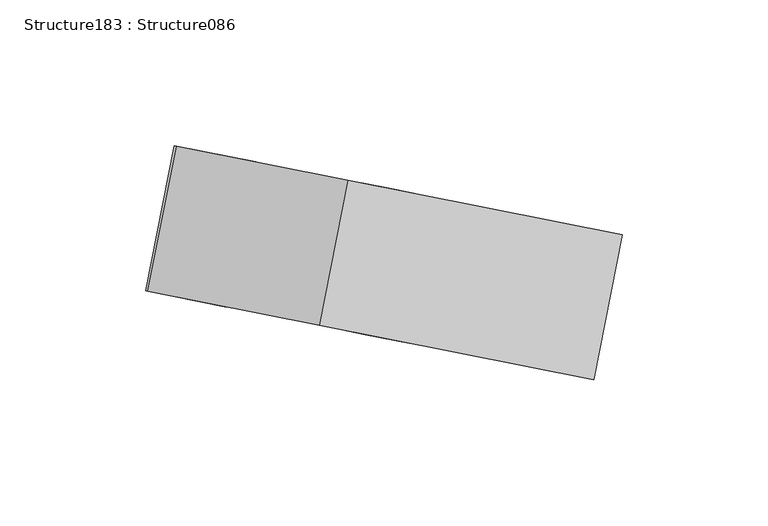
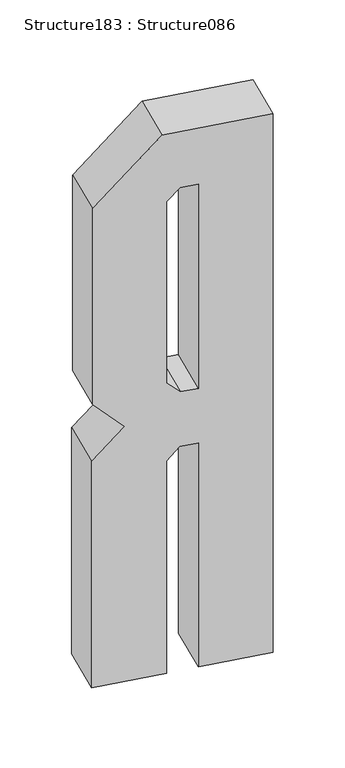
"""IFC4 building model written with IfcOpenShell, lengths in millimetres: proxy geometry, Structure183 : Structure086."""

from ifc_helpers import new_model, si_unit, frame, origin, place, context, project, spatial, polyline, outline, extrude, source, transform, mapped, element, save


def structure183_structure086_f05c0c5b(model_context):
    return source(origin(), model_context, "Body", "SweptSolid", [
        extrude(outline(polyline([(225.8643819, 0.0), (225.8643819, -64.5407118), (13.8227312, -64.5407118), (2.2982141, -76.0652289), (2.2982141, -92.2007628), (225.8643819, -92.2007628), (225.8643819, -156.7268861), (-311.916648, -156.7268861), (-311.916648, -60.6961224), (-251.9962041, -0.7756785), (-56.8607841, -0.7756785), (-28.4303921, -28.4303921), (0.0, 0.0), (225.8643819, 0.0)]), holes=[polyline([(-52.2437186, -92.2007628), (-52.2437186, -76.8327236), (-63.769659, -65.3067832), (-244.3166322, -65.3067832), (-255.8411493, -76.8313003), (-255.8411493, -92.2007628), (-52.2437186, -92.2007628)])]), frame((-2923.2339662, 235046.9068249, 821.1178087), z_axis=(0.19466222296394123, 0.9808703374813295, 0.0), x_axis=(0.0, 0.0, -1.0)), (0.0, 0.0, 1.0), 50.8),
    ])


if __name__ == "__main__":
    model = new_model("IFC4")
    model_context = context("Model", 3, world=origin())
    ifc_project = project(units=[si_unit("LENGTHUNIT", "METRE", prefix="MILLI")], contexts=[model_context])
    site = spatial("IfcSite", under=ifc_project)
    building = spatial("IfcBuilding", under=site)
    placement = place(None, origin())
    structure183_structure086_shape = structure183_structure086_f05c0c5b(model_context)
    element("IfcBuildingElementProxy", 1, Name="Structure183 : Structure086", ObjectType="Structure183 : Structure086", at=placement, inside=building, context=model_context, shape_type="MappedRepresentation", body=[
        mapped(structure183_structure086_shape, transform((0.0, 0.0, 0.0), x_axis=(1.0, 0.0, 0.0), y_axis=(0.0, 1.0, 0.0), z_axis=(0.0, 0.0, 1.0))),
    ])
    save(model, "model.ifc")

# Revit data of these elements
# Type "Structure183 : Structure086"
#   NameOverride = "Structure086"
# Element 1 (IfcBuildingElementProxy, "Structure183 : Structure086")
#   Materials on its faces: "BRUSHED ALUMINUM LETTERING"
# Materials
#   "BRUSHED ALUMINUM LETTERING": class "Unassigned", colour RGB 169 181 186, transparency 0, Cost = 0
